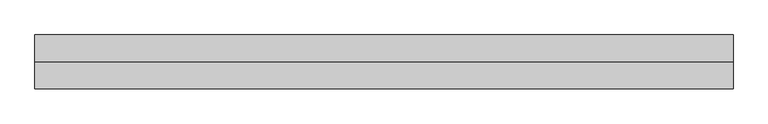
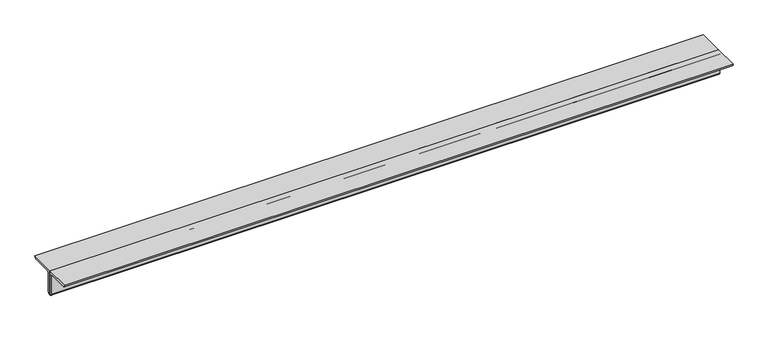
"""IFC4 building model written with IfcOpenShell, lengths in millimetres: member geometry, 0123_Steel Framing_2Ls-KSD3502 : H_SB_AR_S03_2Ls-130x130x12_HBR4."""

from ifc_helpers import new_model, si_unit, point, frame, frame_2d, origin, place, context, project, spatial, polyline, circle_curve, trimmed, segment, composite_curve, outline, extrude, source, transform, mapped, element, save


def member_dd5de35d(model_context):
    return source(origin(), model_context, "Body", "SweptSolid", [
        extrude(outline(composite_curve([segment(polyline([(0.0, 36.4), (130.0, 36.4)]), True, "CONTINUOUS"), segment(trimmed(circle_curve(frame_2d((118.0, 36.4)), 12.0), [point((130.0, 36.4))], [point((118.0, 24.4))], False, "CARTESIAN"), True, "CONTINUOUS"), segment(polyline([(118.0, 24.4), (24.0, 24.4)]), True, "CONTINUOUS"), segment(trimmed(circle_curve(frame_2d((24.0, 12.4)), 12.0), [point((24.0, 24.4))], [point((12.0, 12.4))], True, "CARTESIAN"), True, "CONTINUOUS"), segment(polyline([(12.0, 12.4), (12.0, -81.6)]), True, "CONTINUOUS"), segment(trimmed(circle_curve(frame_2d((0.0, -81.6)), 12.0), [point((12.0, -81.6))], [point((0.0, -93.6))], False, "CARTESIAN"), True, "CONTINUOUS"), segment(polyline([(0.0, -93.6), (0.0, 36.4)]), True, "CONTINUOUS")], self_intersect=False)), frame((-1650.3071495, 0.0, 0.0), z_axis=(1.0, 0.0, 0.0), x_axis=(0.0, 1.0, 0.0)), (0.0, 0.0, 1.0), 3370.5401773),
        extrude(outline(composite_curve([segment(polyline([(0.0, 36.4), (0.0, -93.6)]), True, "CONTINUOUS"), segment(trimmed(circle_curve(frame_2d((0.0, -81.6)), 12.0), [point((0.0, -93.6))], [point((-12.0, -81.6))], False, "CARTESIAN"), True, "CONTINUOUS"), segment(polyline([(-12.0, -81.6), (-12.0, 12.4)]), True, "CONTINUOUS"), segment(trimmed(circle_curve(frame_2d((-24.0, 12.4)), 12.0), [point((-12.0, 12.4))], [point((-24.0, 24.4))], True, "CARTESIAN"), True, "CONTINUOUS"), segment(polyline([(-24.0, 24.4), (-118.0, 24.4)]), True, "CONTINUOUS"), segment(trimmed(circle_curve(frame_2d((-118.0, 36.4)), 12.0), [point((-118.0, 24.4))], [point((-130.0, 36.4))], False, "CARTESIAN"), True, "CONTINUOUS"), segment(polyline([(-130.0, 36.4), (0.0, 36.4)]), True, "CONTINUOUS")], self_intersect=False)), frame((-1650.3071495, 0.0, 0.0), z_axis=(1.0, 0.0, 0.0), x_axis=(0.0, 1.0, 0.0)), (0.0, 0.0, 1.0), 3370.5401773),
    ])


if __name__ == "__main__":
    model = new_model("IFC4")
    model_context = context("Model", 3, world=origin())
    ifc_project = project(units=[si_unit("LENGTHUNIT", "METRE", prefix="MILLI")], contexts=[model_context])
    site = spatial("IfcSite", under=ifc_project)
    building = spatial("IfcBuilding", under=site)
    placement = place(None, origin())
    member_shape = member_dd5de35d(model_context)
    element("IfcMember", 1, ObjectType="0123_Steel Framing_2Ls-KSD3502 : H_SB_AR_S03_2Ls-130x130x12_HBR4", at=placement, inside=building, context=model_context, shape_type="MappedRepresentation", body=[
        mapped(member_shape, transform((0.0, 0.0, 0.0), x_axis=(1.0, 0.0, 0.0), y_axis=(0.0, 1.0, 0.0), z_axis=(0.0, 0.0, 1.0))),
    ])
    save(model, "model.ifc")

# Revit data of these elements
# Type "0123_Steel Framing_2Ls-KSD3502 : H_SB_AR_S03_2Ls-130x130x12_HBR4"
#   Type Mark = "HBR4"
#   Assembly Code = "B10"
#   Legs = "SLBB"
#   W = 8.97
#   Perimeter = 1.04 m²/m
#   Nominal Weight = 46.80 kgf/m
#   Length [instance default] = 1000 mm
#   Space = 0 mm
#   b = 130 mm
#   d = 130 mm
#   t = 12 mm
#   y = 36.4 mm
#   A = 0.005952 m²
#   Structural Material [instance default] = Steel ASTM A36
# Element 1 (IfcMember, "0123_Steel Framing_2Ls-KSD3502 : H_SB_AR_S03_2Ls-130x130x12_HBR4")
#   Materials on its faces: "Steel ASTM A36"
# Materials
#   "Steel ASTM A36": class "Metal", colour RGB 199 199 199, transparency 0, Description = "Structural steel, ASTM A36 Grade B, mill finish", Cost = 0
